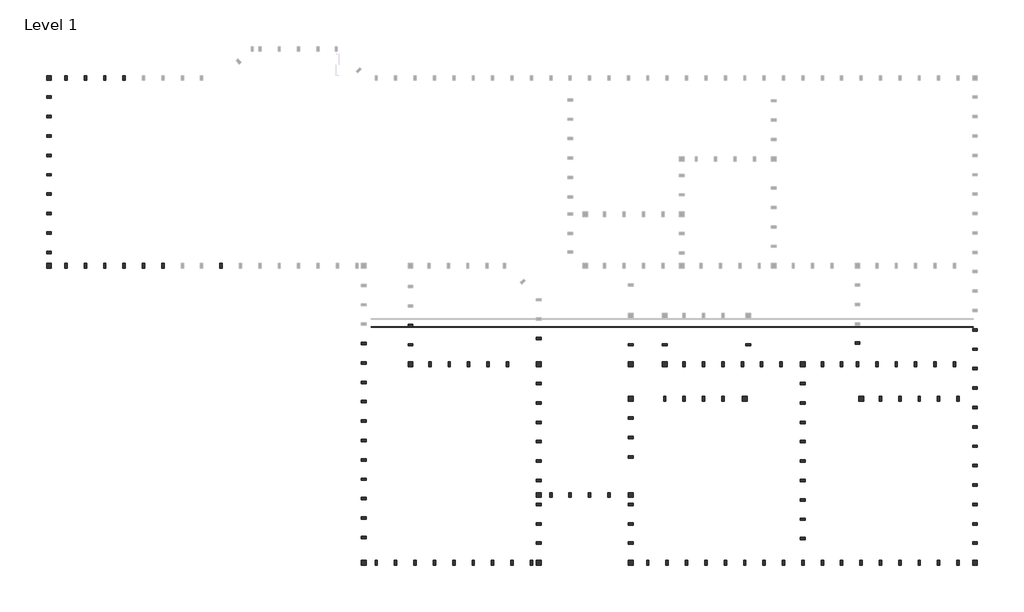
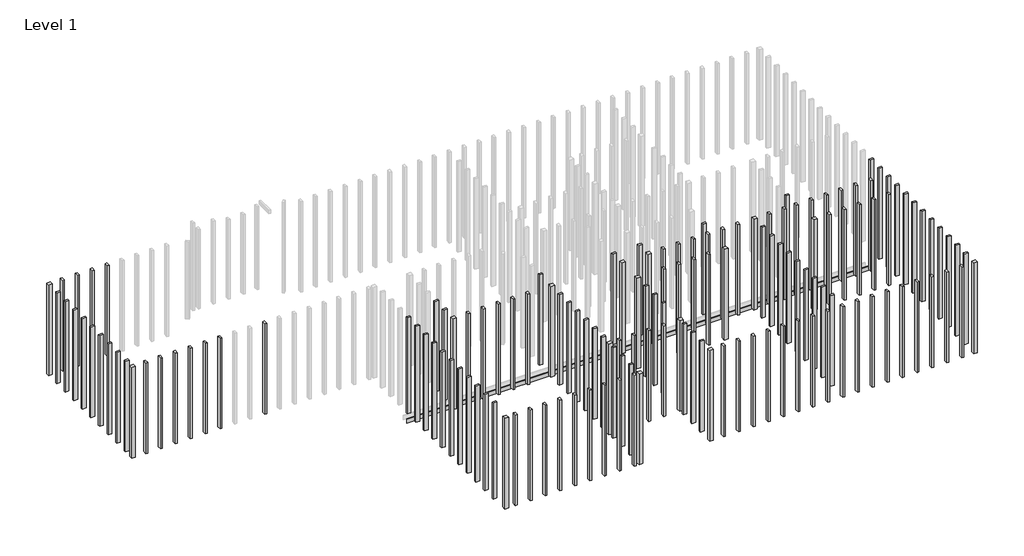
# One storey, part 1 of 2: 148 columns, 1 beam.
# Revit data of these elements (continued)
# Elements 105, 106, 107, 108, 109, 110, 111, 112, 113, 114, 115, 116, 117, 118, 119, 120 (IfcColumn, "Timber-Column : BLDG 6241 Wall Struds 4\"x4\"")
#   Comments = ""
#   Structural Material = Softwood, Lumber
#   Phase Created = New Construction
#   Materials on its faces: "Softwood, Lumber"
# Materials
#   "Softwood, Lumber": class "Wood", colour RGB 223 192 134, transparency 0, Description = "Pinus Echinata", Cost = 0
#   "Plywood, Sheathing": class "Wood", colour RGB 212 179 113, transparency 0, Description = "Plywood, sheathing grade", Cost = 0
